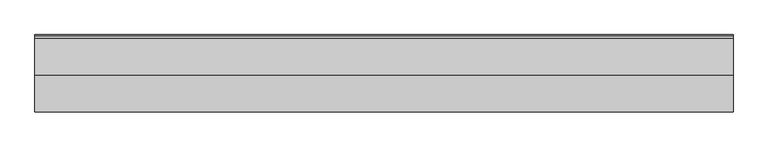
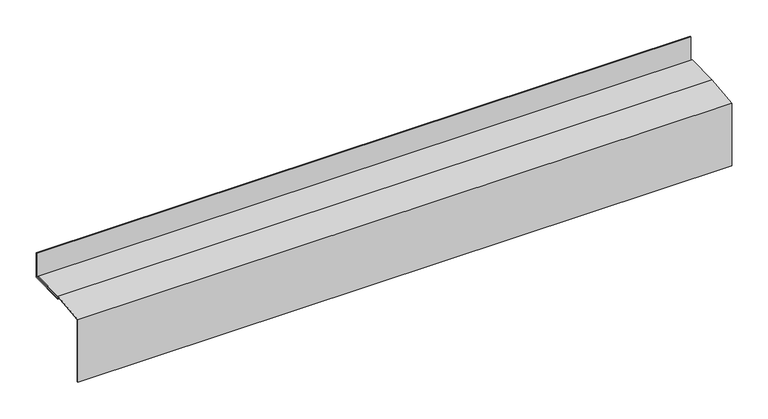
"""IFC4 building model written with IfcOpenShell, lengths in millimetres: proxy geometry, Generic Models 7:Generic Models 1:7:Generic Models 1:7 : Generic Models 7:Generic Models 1:337419:5 : Generic Models 7:Generic Models 1:7:Generic Models 1:7 : Generic Models 7:Generic Models 1:337419:315055."""

from ifc_helpers import new_model, si_unit, origin, place, context, project, spatial, faceted_brep, source, transform, mapped, element, save


def generic_models_f1a9c836(model_context):
    return source(origin(), model_context, "Body", "Brep", [
        faceted_brep([(592758.9138536, -579144.4191956, -81.7582633), (592758.9138536, -579144.4191956, 22.8699913), (592758.9138536, -579090.4900272, 28.8582208), (592758.9138536, -579036.0276865, 28.8582208), (592758.9138536, -579036.0276865, 30.4457208), (592758.9138536, -579090.5778942, 30.4457208), (592758.9138536, -579146.0066956, 24.2909738), (592758.9138536, -579146.0066956, -81.7582633), (591714.0570845, -579144.4191956, -81.7582633), (591714.0570845, -579146.0066956, -81.7582633), (591714.0570845, -579146.0066956, 22.420253), (591714.0570845, -579146.0066956, 24.2909738), (591714.0570845, -579090.5778942, 30.4457208), (591714.0570845, -579036.0276865, 30.4457208), (591714.0570845, -579036.0276865, 28.8582208), (591714.0570845, -579090.4900272, 28.8582208), (591714.0570845, -579144.4191956, 22.8699913), (591714.0570845, -579144.4191956, 20.9992705)], [[[0, 1, 2, 3, 4, 5, 6, 7]], [[8, 9, 10, 11, 12, 13, 14, 15, 16, 17]], [[1, 0, 8, 17, 16]], [[7, 6, 11, 10, 9]], [[0, 7, 9, 8]], [[3, 2, 15, 14]], [[5, 4, 13, 12]], [[6, 5, 12, 11]], [[4, 3, 14, 13]], [[2, 1, 16, 15]]]),
        faceted_brep([(592758.9138536, -579090.7820091, 27.0981204), (592758.9138536, -579090.7820091, 25.5106204), (592758.9138536, -579030.283904, 25.5106204), (592758.9138536, -579030.283904, 67.1553788), (592758.9138536, -579031.871404, 67.1553788), (592758.9138536, -579031.871404, 27.0981204), (591714.0570845, -579090.7820091, 27.0981204), (591714.0570845, -579031.871404, 27.0981204), (591714.0570845, -579031.871404, 67.1553788), (591714.0570845, -579030.283904, 67.1553788), (591714.0570845, -579030.283904, 25.5106204), (591714.0570845, -579090.7820091, 25.5106204)], [[[0, 1, 2, 3, 4, 5]], [[6, 7, 8, 9, 10, 11]], [[1, 0, 6, 11]], [[2, 1, 11, 10]], [[3, 2, 10, 9]], [[4, 3, 9, 8]], [[5, 4, 8, 7]], [[0, 5, 7, 6]]]),
    ])


if __name__ == "__main__":
    model = new_model("IFC4")
    model_context = context("Model", 3, world=origin())
    ifc_project = project(units=[si_unit("LENGTHUNIT", "METRE", prefix="MILLI")], contexts=[model_context])
    site = spatial("IfcSite", under=ifc_project)
    building = spatial("IfcBuilding", under=site)
    placement = place(None, origin())
    generic_models_shape = generic_models_f1a9c836(model_context)
    element("IfcBuildingElementProxy", 1, Name="Generic Models 7:Generic Models 1:7:Generic Models 1:7 : Generic Models 7:Generic Models 1:337419:5 : Generic Models 7:Generic Models 1:7:Generic Models 1:7 : Generic Models 7:Generic Models 1:337419:315055", ObjectType="Generic Models 7:Generic Models 1:7:Generic Models 1:7 : Generic Models 7:Generic Models 1:337419:5 : Generic Models 7:Generic Models 1:7:Generic Models 1:7 : Generic Models 7:Generic Models 1:337419:315055", at=placement, inside=building, context=model_context, shape_type="MappedRepresentation", body=[
        mapped(generic_models_shape, transform((0.0, 0.0, 0.0), x_axis=(1.0, 0.0, 0.0), y_axis=(0.0, 1.0, 0.0), z_axis=(0.0, 0.0, 1.0))),
    ])
    save(model, "model.ifc")

# Revit data of these elements
# Type "Generic Models 7:Generic Models 1:7:Generic Models 1:7 : Generic Models 7:Generic Models 1:337419:5 : Generic Models 7:Generic Models 1:7:Generic Models 1:7 : Generic Models 7:Generic Models 1:337419:315055"
#   NameOverride = "Generic Models 7:Generic Models 1:7:Generic Models 1:7 : Generic Models 7:Generic Models 1:337419:315055"
#   ObjectTypeOverride = "Generic Models 1:7 : Generic Models 7:Generic Models 1:337419"
#   Reference = "Generic Models 1"
#   Tag = "315055"
# Element 1 (IfcBuildingElementProxy, "Generic Models 7:Generic Models 1:7:Generic Models 1:7 : Generic Models 7:Generic Models 1:337419:5 : Generic Models 7:Generic Models 1:7:Generic Models 1:7 : Generic Models 7:Generic Models 1:337419:315055")
#   Materials on its faces: "ANODIZED ALUM. FLASHING - MATCH STOREFRONT (ALIGN WITH OTHER WALL ASSEMBLIES)"
# Materials
#   "ANODIZED ALUM. FLASHING - MATCH STOREFRONT (ALIGN WITH OTHER WALL ASSEMBLIES)": class "Unassigned", colour RGB 210 209 208, transparency 0, Cost = 0
